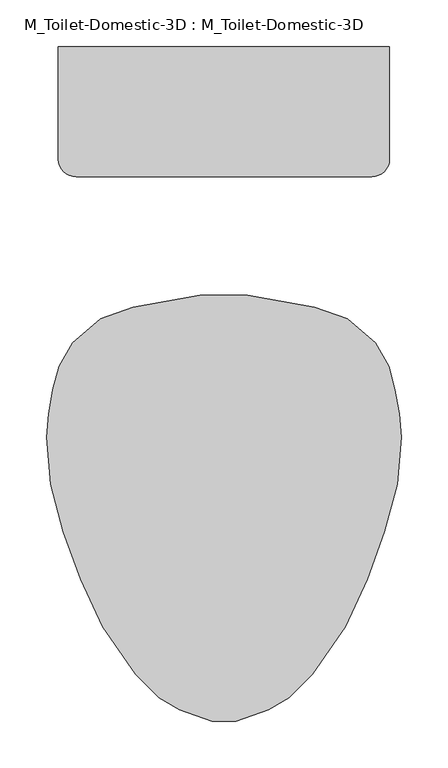
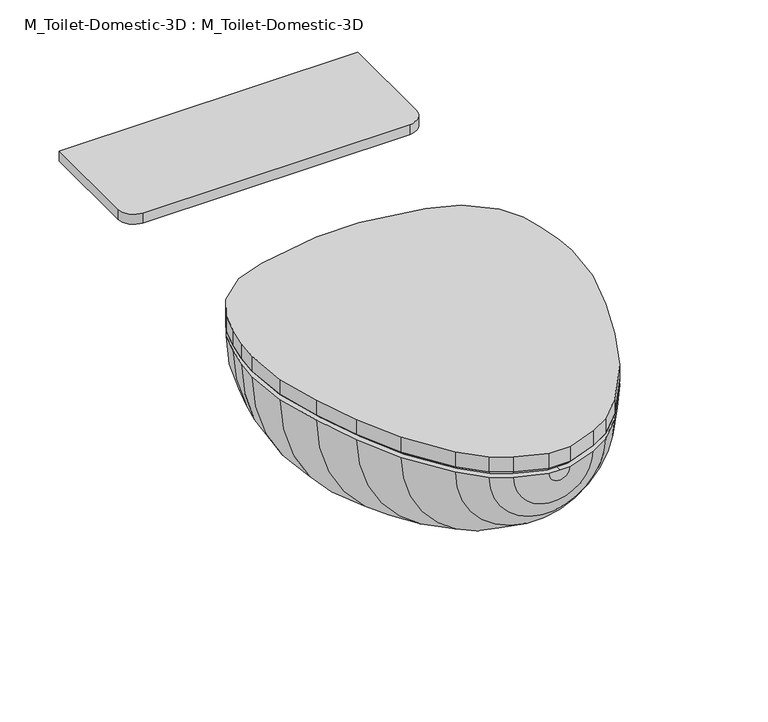
"""IFC4 building model written with IfcOpenShell, lengths in millimetres: flow terminal geometry, M_Toilet-Domestic-3D : M_Toilet-Domestic-3D."""

from ifc_helpers import new_model, si_unit, point, frame, frame_2d, origin, place, context, project, spatial, polyline, circle_curve, trimmed, segment, composite_curve, outline, extrude, faceted_brep, source, transform, mapped, element, save
from ifc_brep_helpers import plane_surface, revolved_surface, advanced_brep


def m_toilet_domestic_3d_m_toilet_domestic_3d_183bbd19(model_context):
    return source(origin(), model_context, "Body", "SolidModel", [
        advanced_brep(
        [(-25.4, 152.4, 361.95), (-97.4252791, 139.7, 361.95), (-132.3182423, 127.0, 361.95), (-162.5887836, 101.6, 361.95), (-176.9845865, 76.2, 361.95), (-183.790496, 50.8, 361.95), (-188.2862441, 25.3033453, 361.95), (-190.5, 0.0, 361.95), (-186.0724883, -50.6066907, 361.95), (-172.4088722, -101.6, 361.95), (-153.9191843, -152.4, 361.95), (-130.2307553, -203.2, 361.95), (-94.9900085, -254.0, 361.95), (-69.5900085, -279.4, 361.95), (-47.5929632, -292.1, 361.95), (-12.7, -304.8, 361.95), (0.0, -304.8, 361.95), (0.0, -284.592034, 361.95), (-12.5224565, -284.592034, 361.95), (-39.5113323, -274.7688865, 361.95), (-58.4178985, -263.8531754, 361.95), (-79.2146703, -243.0564036, 361.95), (-114.0255101, -192.8761202, 361.95), (-136.654021, -144.3491221, 361.95), (-154.575847, -95.1093097, 361.95), (-167.7238545, -46.0402777, 361.95), (-171.5645445, -2.1409906, 361.95), (-169.3087351, 23.6430284, 361.95), (-165.101298, 47.5045901, 361.95), (-159.5484355, 68.2281551, 361.95), (-146.1085923, 90.5605136, 361.95), (-121.9980886, 110.7916284, 361.95), (-94.1172813, 120.9394123, 361.95), (-22.0920022, 133.6394123, 361.95), (0.0, 133.6394123, 361.95), (0.0, 152.4, 361.95), (25.4, 152.4, 361.95), (22.0920022, 133.6394123, 361.95), (94.1172813, 120.9394123, 361.95), (121.9980886, 110.7916284, 361.95), (146.1085923, 90.5605136, 361.95), (159.5484355, 68.2281551, 361.95), (165.101298, 47.5045901, 361.95), (169.3087351, 23.6430284, 361.95), (171.5645445, -2.1409906, 361.95), (167.7238545, -46.0402777, 361.95), (154.575847, -95.1093097, 361.95), (136.654021, -144.3491221, 361.95), (114.0255101, -192.8761202, 361.95), (79.2146703, -243.0564036, 361.95), (58.4178985, -263.8531754, 361.95), (39.5113323, -274.7688865, 361.95), (12.5224565, -284.592034, 361.95), (12.7, -304.8, 361.95), (47.5929632, -292.1, 361.95), (69.5900085, -279.4, 361.95), (94.9900085, -254.0, 361.95), (130.2307553, -203.2, 361.95), (153.9191843, -152.4, 361.95), (172.4088722, -101.6, 361.95), (186.0724883, -50.6066907, 361.95), (190.5, 0.0, 361.95), (188.2862441, 25.3033453, 361.95), (183.790496, 50.8, 361.95), (176.9845865, 76.2, 361.95), (162.5887836, 101.6, 361.95), (132.3182423, 127.0, 361.95), (97.4252791, 139.7, 361.95)],
        [
            (0, 1),
            (1, 2),
            (2, 3),
            (3, 4),
            (4, 5),
            (5, 6),
            (6, 7),
            (7, 8),
            (8, 9),
            (9, 10),
            (10, 11),
            (11, 12),
            (12, 13),
            (13, 14),
            (14, 15),
            (15, 16),
            (16, 17),
            (17, 18),
            (18, 19),
            (19, 20),
            (20, 21),
            (21, 22),
            (22, 23),
            (23, 24),
            (24, 25),
            (25, 26),
            (26, 27),
            (27, 28),
            (28, 29),
            (29, 30),
            (30, 31),
            (31, 32),
            (32, 33),
            (33, 34),
            (34, 35),
            (35, 0),
            (36, 35),
            (34, 37),
            (37, 38),
            (38, 39),
            (39, 40),
            (40, 41),
            (41, 42),
            (42, 43),
            (43, 44),
            (44, 45),
            (45, 46),
            (46, 47),
            (47, 48),
            (48, 49),
            (49, 50),
            (50, 51),
            (51, 52),
            (52, 17),
            (16, 53),
            (53, 54),
            (54, 55),
            (55, 56),
            (56, 57),
            (57, 58),
            (58, 59),
            (59, 60),
            (60, 61),
            (61, 62),
            (62, 63),
            (63, 64),
            (64, 65),
            (65, 66),
            (66, 67),
            (67, 36),
            (67, 1, circle_curve(frame((0.0, 139.7, 361.95), z_axis=(0.0, 1.0, 0.0), x_axis=(-1.0, 0.0, 0.0)), 97.4252791)),
            (0, 36, circle_curve(frame((0.0, 152.4, 361.95), z_axis=(0.0, -1.0, 0.0), x_axis=(-1.0, 0.0, 0.0)), 25.4)),
            (66, 2, circle_curve(frame((0.0, 127.0, 361.95), z_axis=(0.0, 1.0, 0.0), x_axis=(-1.0, 0.0, 0.0)), 132.3182423)),
            (65, 3, circle_curve(frame((0.0, 101.6, 361.95), z_axis=(0.0, 1.0, 0.0), x_axis=(-1.0, 0.0, 0.0)), 162.5887836)),
            (64, 4, circle_curve(frame((0.0, 76.2, 361.95), z_axis=(0.0, 1.0, 0.0), x_axis=(-1.0, 0.0, 0.0)), 176.9845865)),
            (63, 5, circle_curve(frame((0.0, 50.8, 361.95), z_axis=(0.0, 1.0, 0.0), x_axis=(-1.0, 0.0, 0.0)), 183.790496)),
            (62, 6, circle_curve(frame((0.0, 25.3033453, 361.95), z_axis=(0.0, 1.0, 0.0), x_axis=(-1.0, 0.0, 0.0)), 188.2862441)),
            (61, 7, circle_curve(frame((0.0, 0.0, 361.95), z_axis=(0.0, 1.0, 0.0), x_axis=(-1.0, 0.0, 0.0)), 190.5)),
            (60, 8, circle_curve(frame((0.0, -50.6066907, 361.95), z_axis=(0.0, 1.0, 0.0), x_axis=(-1.0, 0.0, 0.0)), 186.0724883)),
            (59, 9, circle_curve(frame((0.0, -101.6, 361.95), z_axis=(0.0, 1.0, 0.0), x_axis=(-1.0, 0.0, 0.0)), 172.4088722)),
            (58, 10, circle_curve(frame((0.0, -152.4, 361.95), z_axis=(0.0, 1.0, 0.0), x_axis=(-1.0, 0.0, 0.0)), 153.9191843)),
            (57, 11, circle_curve(frame((0.0, -203.2, 361.95), z_axis=(0.0, 1.0, 0.0), x_axis=(-1.0, 0.0, 0.0)), 130.2307553)),
            (56, 12, circle_curve(frame((0.0, -254.0, 361.95), z_axis=(0.0, 1.0, 0.0), x_axis=(-1.0, 0.0, 0.0)), 94.9900085)),
            (55, 13, circle_curve(frame((0.0, -279.4, 361.95), z_axis=(0.0, 1.0, 0.0), x_axis=(-1.0, 0.0, 0.0)), 69.5900085)),
            (54, 14, circle_curve(frame((0.0, -292.1, 361.95), z_axis=(0.0, 1.0, 0.0), x_axis=(-1.0, 0.0, 0.0)), 47.5929632)),
            (53, 15, circle_curve(frame((0.0, -304.8, 361.95), z_axis=(0.0, 1.0, 0.0), x_axis=(-1.0, 0.0, 0.0)), 12.7)),
            (52, 18, circle_curve(frame((0.0, -284.592034, 361.95), z_axis=(0.0, 1.0, 0.0), x_axis=(-1.0, 0.0, 0.0)), 12.5224565)),
            (51, 19, circle_curve(frame((0.0, -274.7688865, 361.95), z_axis=(0.0, 1.0, 0.0), x_axis=(-1.0, 0.0, 0.0)), 39.5113323)),
            (50, 20, circle_curve(frame((0.0, -263.8531754, 361.95), z_axis=(0.0, 1.0, 0.0), x_axis=(-1.0, 0.0, 0.0)), 58.4178985)),
            (49, 21, circle_curve(frame((0.0, -243.0564036, 361.95), z_axis=(0.0, 1.0, 0.0), x_axis=(-1.0, 0.0, 0.0)), 79.2146703)),
            (48, 22, circle_curve(frame((0.0, -192.8761202, 361.95), z_axis=(0.0, 1.0, 0.0), x_axis=(-1.0, 0.0, 0.0)), 114.0255101)),
            (47, 23, circle_curve(frame((0.0, -144.3491221, 361.95), z_axis=(0.0, 1.0, 0.0), x_axis=(-1.0, 0.0, 0.0)), 136.654021)),
            (46, 24, circle_curve(frame((0.0, -95.1093097, 361.95), z_axis=(0.0, 1.0, 0.0), x_axis=(-1.0, 0.0, 0.0)), 154.575847)),
            (45, 25, circle_curve(frame((0.0, -46.0402777, 361.95), z_axis=(0.0, 1.0, 0.0), x_axis=(-1.0, 0.0, 0.0)), 167.7238545)),
            (44, 26, circle_curve(frame((0.0, -2.1409906, 361.95), z_axis=(0.0, 1.0, 0.0), x_axis=(-1.0, 0.0, 0.0)), 171.5645445)),
            (43, 27, circle_curve(frame((0.0, 23.6430284, 361.95), z_axis=(0.0, 1.0, 0.0), x_axis=(-1.0, 0.0, 0.0)), 169.3087351)),
            (42, 28, circle_curve(frame((0.0, 47.5045901, 361.95), z_axis=(0.0, 1.0, 0.0), x_axis=(-1.0, 0.0, 0.0)), 165.101298)),
            (41, 29, circle_curve(frame((0.0, 68.2281551, 361.95), z_axis=(0.0, 1.0, 0.0), x_axis=(-1.0, 0.0, 0.0)), 159.5484355)),
            (40, 30, circle_curve(frame((0.0, 90.5605136, 361.95), z_axis=(0.0, 1.0, 0.0), x_axis=(-1.0, 0.0, 0.0)), 146.1085923)),
            (39, 31, circle_curve(frame((0.0, 110.7916284, 361.95), z_axis=(0.0, 1.0, 0.0), x_axis=(-1.0, 0.0, 0.0)), 121.9980886)),
            (38, 32, circle_curve(frame((0.0, 120.9394123, 361.95), z_axis=(0.0, 1.0, 0.0), x_axis=(-1.0, 0.0, 0.0)), 94.1172813)),
            (37, 33, circle_curve(frame((0.0, 133.6394123, 361.95), z_axis=(0.0, 1.0, 0.0), x_axis=(-1.0, 0.0, 0.0)), 22.0920022)),
        ],
        [
            plane_surface(frame((0.0, 175.1599017, 361.95), z_axis=(0.0, 0.0, 1.0), x_axis=(-1.0, 0.0, 0.0))),
            plane_surface(frame((0.0, 175.1599017, 361.95), z_axis=(0.0, 0.0, 1.0), x_axis=(1.0, 0.0, 0.0))),
            revolved_surface(polyline([(-25.4, 152.4, 361.95), (-97.4252791, 139.7, 361.95)]), (0.0, 175.1599017, 361.95), (0.0, -1.0, 0.0)),
            revolved_surface(polyline([(-97.4252791, 139.7, 361.95), (-132.3182423, 127.0, 361.95)]), (0.0, 175.1599017, 361.95), (0.0, -1.0, 0.0)),
            revolved_surface(polyline([(-132.3182423, 127.0, 361.95), (-162.5887836, 101.6, 361.95)]), (0.0, 175.1599017, 361.95), (0.0, -1.0, 0.0)),
            revolved_surface(polyline([(-162.5887836, 101.6, 361.95), (-176.9845865, 76.2, 361.95)]), (0.0, 175.1599017, 361.95), (0.0, -1.0, 0.0)),
            revolved_surface(polyline([(-176.9845865, 76.2, 361.95), (-183.790496, 50.8, 361.95)]), (0.0, 175.1599017, 361.95), (0.0, -1.0, 0.0)),
            revolved_surface(polyline([(-183.790496, 50.8, 361.95), (-188.2862441, 25.3033453, 361.95)]), (0.0, 175.1599017, 361.95), (0.0, -1.0, 0.0)),
            revolved_surface(polyline([(-188.2862441, 25.3033453, 361.95), (-190.5, 0.0, 361.95)]), (0.0, 175.1599017, 361.95), (0.0, -1.0, 0.0)),
            revolved_surface(polyline([(-190.5, 0.0, 361.95), (-186.0724883, -50.6066907, 361.95)]), (0.0, 175.1599017, 361.95), (0.0, -1.0, 0.0)),
            revolved_surface(polyline([(-186.0724883, -50.6066907, 361.95), (-172.4088722, -101.6, 361.95)]), (0.0, 175.1599017, 361.95), (0.0, -1.0, 0.0)),
            revolved_surface(polyline([(-172.4088722, -101.6, 361.95), (-153.9191843, -152.4, 361.95)]), (0.0, 175.1599017, 361.95), (0.0, -1.0, 0.0)),
            revolved_surface(polyline([(-153.9191843, -152.4, 361.95), (-130.2307553, -203.2, 361.95)]), (0.0, 175.1599017, 361.95), (0.0, -1.0, 0.0)),
            revolved_surface(polyline([(-130.2307553, -203.2, 361.95), (-94.9900085, -254.0, 361.95)]), (0.0, 175.1599017, 361.95), (0.0, -1.0, 0.0)),
            revolved_surface(polyline([(-94.9900085, -254.0, 361.95), (-69.5900085, -279.4, 361.95)]), (0.0, 175.1599017, 361.95), (0.0, -1.0, 0.0)),
            revolved_surface(polyline([(-69.5900085, -279.4, 361.95), (-47.5929632, -292.1, 361.95)]), (0.0, 175.1599017, 361.95), (0.0, -1.0, 0.0)),
            revolved_surface(polyline([(-47.5929632, -292.1, 361.95), (-12.7, -304.8, 361.95)]), (0.0, 175.1599017, 361.95), (0.0, -1.0, 0.0)),
            plane_surface(frame((0.0, -304.8, 361.95), z_axis=(0.0, -1.0, 0.0), x_axis=(-1.0, 0.0, 0.0))),
            plane_surface(frame((0.0, -284.592034, 361.95), z_axis=(0.0, 1.0, 0.0), x_axis=(-1.0, 0.0, 0.0))),
            revolved_surface(polyline([(-12.5224565, -284.592034, 361.95), (-39.5113323, -274.7688865, 361.95)]), (0.0, 175.1599017, 361.95), (0.0, -1.0, 0.0)),
            revolved_surface(polyline([(-39.5113323, -274.7688865, 361.95), (-58.4178985, -263.8531754, 361.95)]), (0.0, 175.1599017, 361.95), (0.0, -1.0, 0.0)),
            revolved_surface(polyline([(-58.4178985, -263.8531754, 361.95), (-79.2146703, -243.0564036, 361.95)]), (0.0, 175.1599017, 361.95), (0.0, -1.0, 0.0)),
            revolved_surface(polyline([(-79.2146703, -243.0564036, 361.95), (-114.0255101, -192.8761202, 361.95)]), (0.0, 175.1599017, 361.95), (0.0, -1.0, 0.0)),
            revolved_surface(polyline([(-114.0255101, -192.8761202, 361.95), (-136.654021, -144.3491221, 361.95)]), (0.0, 175.1599017, 361.95), (0.0, -1.0, 0.0)),
            revolved_surface(polyline([(-136.654021, -144.3491221, 361.95), (-154.575847, -95.1093097, 361.95)]), (0.0, 175.1599017, 361.95), (0.0, -1.0, 0.0)),
            revolved_surface(polyline([(-154.575847, -95.1093097, 361.95), (-167.7238545, -46.0402777, 361.95)]), (0.0, 175.1599017, 361.95), (0.0, -1.0, 0.0)),
            revolved_surface(polyline([(-167.7238545, -46.0402777, 361.95), (-171.5645445, -2.1409906, 361.95)]), (0.0, 175.1599017, 361.95), (0.0, -1.0, 0.0)),
            revolved_surface(polyline([(-171.5645445, -2.1409906, 361.95), (-169.3087351, 23.6430284, 361.95)]), (0.0, 175.1599017, 361.95), (0.0, -1.0, 0.0)),
            revolved_surface(polyline([(-169.3087351, 23.6430284, 361.95), (-165.101298, 47.5045901, 361.95)]), (0.0, 175.1599017, 361.95), (0.0, -1.0, 0.0)),
            revolved_surface(polyline([(-165.101298, 47.5045901, 361.95), (-159.5484355, 68.2281551, 361.95)]), (0.0, 175.1599017, 361.95), (0.0, -1.0, 0.0)),
            revolved_surface(polyline([(-159.5484355, 68.2281551, 361.95), (-146.1085923, 90.5605136, 361.95)]), (0.0, 175.1599017, 361.95), (0.0, -1.0, 0.0)),
            revolved_surface(polyline([(-146.1085923, 90.5605136, 361.95), (-121.9980886, 110.7916284, 361.95)]), (0.0, 175.1599017, 361.95), (0.0, -1.0, 0.0)),
            revolved_surface(polyline([(-121.9980886, 110.7916284, 361.95), (-94.1172813, 120.9394123, 361.95)]), (0.0, 175.1599017, 361.95), (0.0, -1.0, 0.0)),
            revolved_surface(polyline([(-94.1172813, 120.9394123, 361.95), (-22.0920022, 133.6394123, 361.95)]), (0.0, 175.1599017, 361.95), (0.0, -1.0, 0.0)),
            plane_surface(frame((0.0, 133.6394123, 361.95), z_axis=(0.0, -1.0, 0.0), x_axis=(-1.0, 0.0, 0.0))),
            plane_surface(frame((0.0, 152.4, 361.95), z_axis=(0.0, 1.0, 0.0), x_axis=(-1.0, 0.0, 0.0))),
        ],
        [
            (0, [[1, 2, 3, 4, 5, 6, 7, 8, 9, 10, 11, 12, 13, 14, 15, 16, 17, 18, 19, 20, 21, 22, 23, 24, 25, 26, 27, 28, 29, 30, 31, 32, 33, 34, 35, 36]]),
            (1, [[37, -35, 38, 39, 40, 41, 42, 43, 44, 45, 46, 47, 48, 49, 50, 51, 52, 53, 54, -17, 55, 56, 57, 58, 59, 60, 61, 62, 63, 64, 65, 66, 67, 68, 69, 70]]),
            (2, [[71, -1, 72, -70]]),
            (3, [[73, -2, -71, -69]]),
            (4, [[74, -3, -73, -68]]),
            (5, [[75, -4, -74, -67]]),
            (6, [[76, -5, -75, -66]]),
            (7, [[77, -6, -76, -65]]),
            (8, [[78, -7, -77, -64]]),
            (9, [[79, -8, -78, -63]]),
            (10, [[80, -9, -79, -62]]),
            (11, [[81, -10, -80, -61]]),
            (12, [[82, -11, -81, -60]]),
            (13, [[83, -12, -82, -59]]),
            (14, [[84, -13, -83, -58]]),
            (15, [[85, -14, -84, -57]]),
            (16, [[86, -15, -85, -56]]),
            (17, [[-16, -86, -55]]),
            (18, [[87, -18, -54]]),
            (19, [[88, -19, -87, -53]]),
            (20, [[89, -20, -88, -52]]),
            (21, [[90, -21, -89, -51]]),
            (22, [[91, -22, -90, -50]]),
            (23, [[92, -23, -91, -49]]),
            (24, [[93, -24, -92, -48]]),
            (25, [[94, -25, -93, -47]]),
            (26, [[95, -26, -94, -46]]),
            (27, [[96, -27, -95, -45]]),
            (28, [[97, -28, -96, -44]]),
            (29, [[98, -29, -97, -43]]),
            (30, [[99, -30, -98, -42]]),
            (31, [[100, -31, -99, -41]]),
            (32, [[101, -32, -100, -40]]),
            (33, [[102, -33, -101, -39]]),
            (34, [[-34, -102, -38]]),
            (35, [[-72, -36, -37]]),
        ],
    ),
        faceted_brep([(-97.4252791, 139.7, 368.3), (-132.3182423, 127.0, 368.3), (-162.5887836, 101.6, 368.3), (-176.9845865, 76.2, 368.3), (-183.790496, 50.8, 368.3), (-188.2862441, 25.3033453, 368.3), (-190.5, 0.0, 368.3), (-186.0724883, -50.6066907, 368.3), (-172.4088722, -101.6, 368.3), (-153.9191843, -152.4, 368.3), (-130.2307553, -203.2, 368.3), (-94.9900085, -254.0, 368.3), (-69.5900085, -279.4, 368.3), (-47.5929632, -292.1, 368.3), (-12.7, -304.8, 368.3), (12.7, -304.8, 368.3), (47.5929632, -292.1, 368.3), (69.5900085, -279.4, 368.3), (94.9900085, -254.0, 368.3), (130.2307553, -203.2, 368.3), (153.9191843, -152.4, 368.3), (172.4088722, -101.6, 368.3), (186.0724883, -50.6066907, 368.3), (190.5, 0.0, 368.3), (188.2862441, 25.3033453, 368.3), (183.790496, 50.8, 368.3), (176.9845865, 76.2, 368.3), (162.5887836, 101.6, 368.3), (132.3182423, 127.0, 368.3), (97.4252791, 139.7, 368.3), (25.4, 152.4, 368.3), (-25.4, 152.4, 368.3), (-95.7755003, 133.5429415, 361.95), (-24.844447, 146.05, 361.95), (24.844447, 146.05, 361.95), (95.7755003, 133.5429415, 361.95), (129.0942628, 121.4159037, 361.95), (157.6293435, 97.472128, 361.95), (171.060664, 73.773864, 361.95), (177.5851102, 49.4242991, 361.95), (181.9845715, 24.4737144, 361.95), (184.125744, 0.0, 361.95), (179.7950716, -49.4998127, 361.95), (166.347, -99.688699, 361.95), (148.0469602, -149.9676451, 361.95), (124.7045808, -200.0255393, 361.95), (90.0971582, -249.9125941, 361.95), (65.691017, -274.3187354, 361.95), (44.8990862, -286.3229622, 361.95), (11.5803237, -298.45, 361.95), (-11.5803237, -298.45, 361.95), (-44.8990862, -286.3229622, 361.95), (-65.691017, -274.3187354, 361.95), (-90.0971582, -249.9125941, 361.95), (-124.7045808, -200.0255393, 361.95), (-148.0469602, -149.9676451, 361.95), (-166.347, -99.688699, 361.95), (-179.7950716, -49.4998127, 361.95), (-184.125744, 0.0, 361.95), (-181.9845715, 24.4737144, 361.95), (-177.5851102, 49.4242991, 361.95), (-171.060664, 73.773864, 361.95), (-157.6293435, 97.472128, 361.95), (-129.0942628, 121.4159037, 361.95)], [[[0, 1, 2, 3, 4, 5, 6, 7, 8, 9, 10, 11, 12, 13, 14, 15, 16, 17, 18, 19, 20, 21, 22, 23, 24, 25, 26, 27, 28, 29, 30, 31]], [[32, 33, 34, 35, 36, 37, 38, 39, 40, 41, 42, 43, 44, 45, 46, 47, 48, 49, 50, 51, 52, 53, 54, 55, 56, 57, 58, 59, 60, 61, 62, 63]], [[32, 63, 1, 0]], [[63, 62, 2, 1]], [[62, 61, 3, 2]], [[61, 60, 4, 3]], [[60, 59, 5, 4]], [[59, 58, 6, 5]], [[58, 57, 7, 6]], [[57, 56, 8, 7]], [[56, 55, 9, 8]], [[55, 54, 10, 9]], [[54, 53, 11, 10]], [[53, 52, 12, 11]], [[52, 51, 13, 12]], [[51, 50, 14, 13]], [[50, 49, 15, 14]], [[49, 48, 16, 15]], [[48, 47, 17, 16]], [[47, 46, 18, 17]], [[46, 45, 19, 18]], [[45, 44, 20, 19]], [[44, 43, 21, 20]], [[43, 42, 22, 21]], [[42, 41, 23, 22]], [[41, 40, 24, 23]], [[40, 39, 25, 24]], [[39, 38, 26, 25]], [[38, 37, 27, 26]], [[37, 36, 28, 27]], [[36, 35, 29, 28]], [[35, 34, 30, 29]], [[34, 33, 31, 30]], [[33, 32, 0, 31]]]),
        extrude(outline(composite_curve([segment(polyline([(177.8, 419.1), (177.8, 298.45)]), True, "CONTINUOUS"), segment(trimmed(circle_curve(frame_2d((158.75, 298.45)), 19.05), [point((177.8, 298.45))], [point((158.75, 279.4))], False, "CARTESIAN"), True, "CONTINUOUS"), segment(polyline([(158.75, 279.4), (-158.75, 279.4)]), True, "CONTINUOUS"), segment(trimmed(circle_curve(frame_2d((-158.75, 298.45)), 19.05), [point((-158.75, 279.4))], [point((-177.8, 298.45))], False, "CARTESIAN"), True, "CONTINUOUS"), segment(polyline([(-177.8, 298.45), (-177.8, 419.1), (177.8, 419.1)]), True, "CONTINUOUS")], self_intersect=False)), frame((0.0, 0.0, 374.65), z_axis=(0.0, 0.0, 1.0), x_axis=(1.0, 0.0, 0.0)), (0.0, 0.0, 1.0), 12.5681453),
        extrude(outline(polyline([(-162.5887836, 101.6), (-132.3182423, 127.0), (-97.4252791, 139.7), (-25.4, 152.4), (25.4, 152.4), (97.4252791, 139.7), (132.3182423, 127.0), (162.5887836, 101.6), (176.9845865, 76.2), (183.790496, 50.8), (188.2862441, 25.3033453), (190.5, 0.0), (186.0724883, -50.6066907), (172.4088722, -101.6), (153.9191843, -152.4), (130.2307553, -203.2), (94.9900085, -254.0), (69.5900085, -279.4), (47.5929632, -292.1), (12.7, -304.8), (-12.7, -304.8), (-47.5929632, -292.1), (-69.5900085, -279.4), (-94.9900085, -254.0), (-130.2307553, -203.2), (-153.9191843, -152.4), (-172.4088722, -101.6), (-186.0724883, -50.6066907), (-190.5, 0.0), (-188.2862441, 25.3033453), (-183.790496, 50.8), (-176.9845865, 76.2), (-162.5887836, 101.6)])), frame((0.0, 0.0, 368.3), z_axis=(0.0, 0.0, 1.0), x_axis=(1.0, 0.0, 0.0)), (0.0, 0.0, 1.0), 19.05),
    ])


if __name__ == "__main__":
    model = new_model("IFC4")
    model_context = context("Model", 3, world=origin())
    ifc_project = project(units=[si_unit("LENGTHUNIT", "METRE", prefix="MILLI")], contexts=[model_context])
    site = spatial("IfcSite", under=ifc_project)
    building = spatial("IfcBuilding", under=site)
    placement = place(None, origin())
    m_toilet_domestic_3d_m_toilet_domestic_3d_shape = m_toilet_domestic_3d_m_toilet_domestic_3d_183bbd19(model_context)
    element("IfcFlowTerminal", 1, ObjectType="M_Toilet-Domestic-3D : M_Toilet-Domestic-3D", at=placement, inside=building, context=model_context, shape_type="MappedRepresentation", body=[
        mapped(m_toilet_domestic_3d_m_toilet_domestic_3d_shape, transform((0.0, 0.0, 0.0), x_axis=(1.0, 0.0, 0.0), y_axis=(0.0, 1.0, 0.0), z_axis=(0.0, 0.0, 1.0))),
    ])
    save(model, "model.ifc")

# Revit data of these elements
# Type "M_Toilet-Domestic-3D : M_Toilet-Domestic-3D"
#   Bowl/Basin Material = Porcelain, Linen
#   Seat Material = Laminate, Linen, Matte
# Element 1 (IfcFlowTerminal, "M_Toilet-Domestic-3D : M_Toilet-Domestic-3D")
#   Materials on its faces: "Porcelain, Linen", "Laminate, Linen, Matte"
# Materials
#   "Porcelain, Linen": class "Ceramic", colour RGB 249 239 230, transparency 0, Description = "Porcelain, linen", Cost = 0
#   "Laminate, Linen, Matte": class "Plastic", colour RGB 249 239 230, transparency 0, Description = "Plastic Laminate - Linen, Matte", Cost = 0
